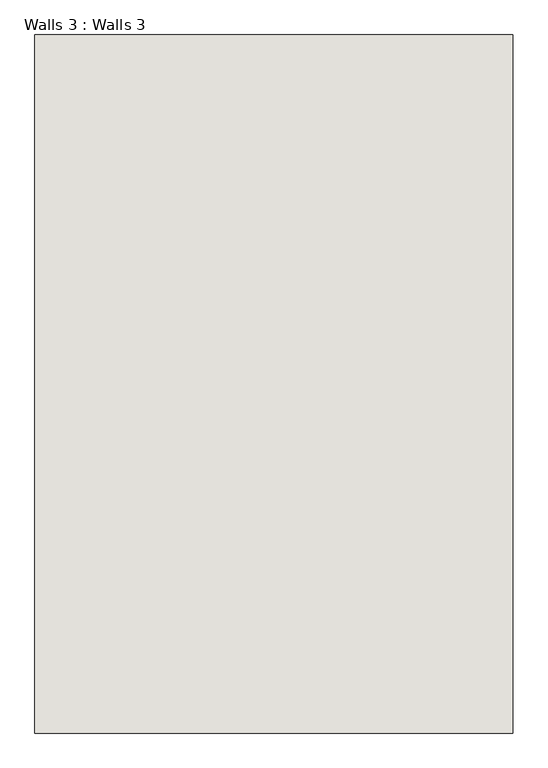
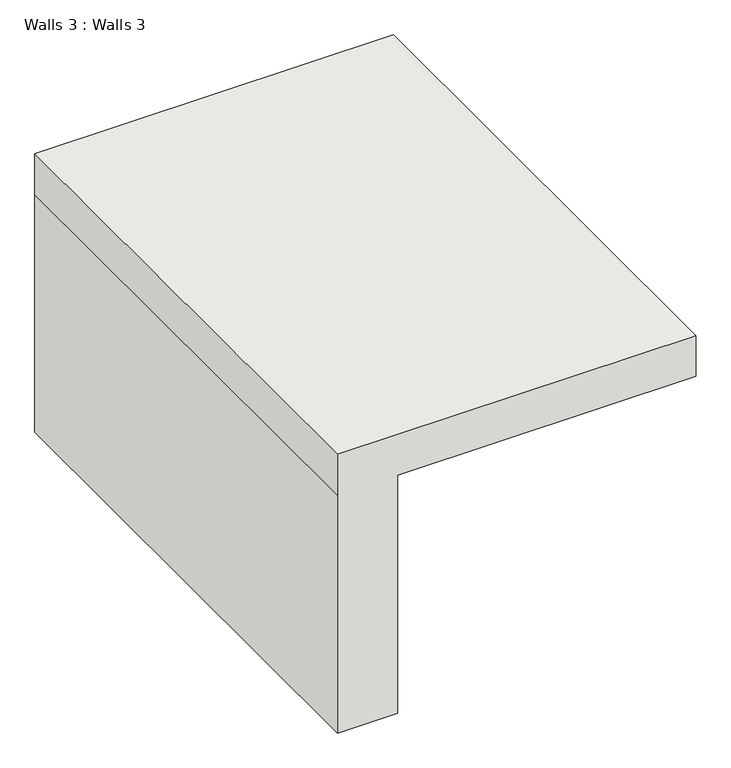
"""IFC4 building model written with IfcOpenShell, lengths in millimetres: wall geometry, Walls 3 : Walls 3."""

from ifc_helpers import new_model, si_unit, frame, origin, place, context, project, spatial, polyline, outline, extrude, source, transform, mapped, element, save


def walls_3_walls_3_c7c27271(model_context):
    return source(origin(), model_context, "Body", "SweptSolid", [
        extrude(outline(polyline([(9000.0, -6925.2511711), (9000.0, -3357.5011711), (9515.0, -3357.5011711), (9515.0, -7639.7511711), (9000.0, -7639.7511711), (6000.0, -7639.7511711), (6000.0, -6925.2511711), (9000.0, -6925.2511711)])), frame((0.0, -9330.1470515, 0.0), z_axis=(0.0, 1.0, 0.0), x_axis=(0.0, 0.0, 1.0)), (0.0, 0.0, 1.0), 6257.25),
    ])


if __name__ == "__main__":
    model = new_model("IFC4")
    model_context = context("Model", 3, world=origin())
    ifc_project = project(units=[si_unit("LENGTHUNIT", "METRE", prefix="MILLI")], contexts=[model_context])
    site = spatial("IfcSite", under=ifc_project)
    building = spatial("IfcBuilding", under=site)
    placement = place(None, origin())
    walls_3_walls_3_shape = walls_3_walls_3_c7c27271(model_context)
    element("IfcWall", 1, ObjectType="Walls 3 : Walls 3", at=placement, inside=building, context=model_context, shape_type="MappedRepresentation", body=[
        mapped(walls_3_walls_3_shape, transform((0.0, 0.0, 0.0), x_axis=(1.0, 0.0, 0.0), y_axis=(0.0, 1.0, 0.0), z_axis=(0.0, 0.0, 1.0))),
    ])
    save(model, "model.ifc")

# Revit data of these elements
# Element 1 (IfcWall, "Walls 3 : Walls 3")
#   Materials on its faces: "Default Wall"
# Materials
#   "Default Wall": class "Miscellaneous", colour RGB 128 128 128, transparency 0, Comments = "Rendering appearance not upgraded ", Cost = 0
